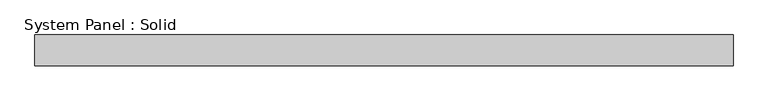
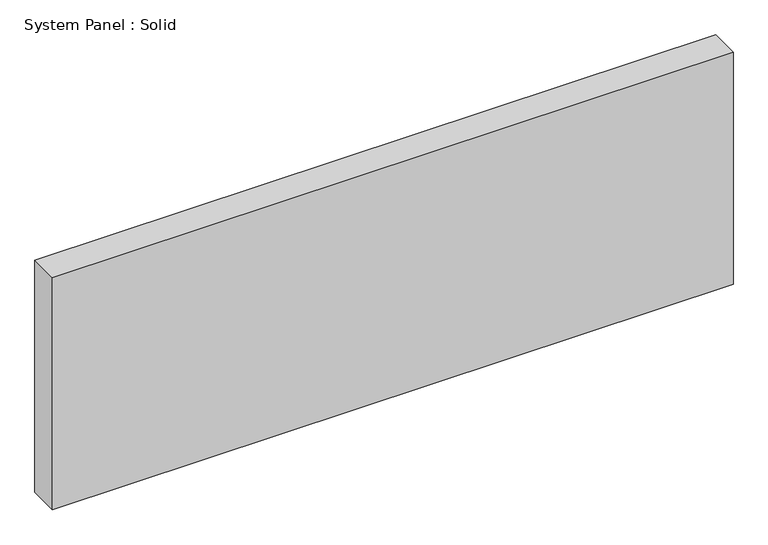
"""IFC4 building model written with IfcOpenShell, lengths in millimetres: plate geometry, System Panel : Solid."""

import ifcopenshell
import ifcopenshell.guid

model = None  # the IFC model being written
_history = None  # IfcOwnerHistory: only IFC2X3 demands one
_inside = {}  # id of a spatial element -> (the spatial element, [elements in it])
_under = {}  # id of a project, library or spatial element -> (it, [spatial elements below it])
_declared = {}  # id of a project -> (the project, [libraries it declares])
_typed = {}  # id of a type object -> (the type object, [elements of that type])
_made_of = {}  # id of a material, layer set ... -> (it, [elements and type objects made of it])


def new_model(schema):
    """Start an empty IFC model of exactly this schema.

    Asked for "IFC4X3", IfcOpenShell would pick the latest addendum, in which some entities
    have other attributes; the version numbers below select the first issue.
    IFC2X3 requires an IfcOwnerHistory on every rooted entity: one is made here for all.
    """
    global model, _history
    if schema == "IFC4X3":
        model = ifcopenshell.file(schema_version=(4, 3, 0, 0))
    else:
        model = ifcopenshell.file(schema=schema)
    _inside.clear()
    _under.clear()
    _declared.clear()
    _typed.clear()
    _made_of.clear()
    _history = None
    if model.schema == "IFC2X3":
        org = make("IfcOrganization", Name="unknown")
        user = make(
            "IfcPersonAndOrganization",
            ThePerson=make("IfcPerson", FamilyName="unknown"),
            TheOrganization=org,
        )
        app = make(
            "IfcApplication",
            ApplicationDeveloper=org,
            Version="unknown",
            ApplicationFullName="unknown",
            ApplicationIdentifier="unknown",
        )
        _history = make(
            "IfcOwnerHistory",
            OwningUser=user,
            OwningApplication=app,
            ChangeAction="ADDED",
            CreationDate=0,
        )
    return model


def make(cls, **values):
    """One entity of the class cls with the attributes given. An attribute that is None is left unset."""
    return model.create_entity(
        cls, **{name: value for name, value in values.items() if value is not None}
    )


def rooted(cls, **values):
    """An entity with a GlobalId (a new one), such as an element, a storey or a relation."""
    return make(cls, GlobalId=ifcopenshell.guid.new(), OwnerHistory=_history, **values)


def si_unit(unit_type, name, prefix=None):
    """IfcSIUnit, for example si_unit("LENGTHUNIT", "METRE", prefix="MILLI")."""
    return make("IfcSIUnit", UnitType=unit_type, Prefix=prefix, Name=name)


def assignment(units):
    """IfcUnitAssignment: the units of a project."""
    return None if units is None else make("IfcUnitAssignment", Units=units)


def point(xyz):
    """IfcCartesianPoint."""
    return None if xyz is None else make("IfcCartesianPoint", Coordinates=xyz)


def direction(xyz):
    """IfcDirection."""
    return None if xyz is None else make("IfcDirection", DirectionRatios=xyz)


def frame(location, z_axis=None, x_axis=None):
    """IfcAxis2Placement3D, a coordinate frame: its origin and axes. An axis left out is left unset."""
    return make(
        "IfcAxis2Placement3D",
        Location=point(location),
        Axis=direction(z_axis),
        RefDirection=direction(x_axis),
    )


def origin():
    """The frame at (0, 0, 0) with its axes left unset."""
    return frame((0.0, 0.0, 0.0))


def origin_with_axes():
    """The frame at (0, 0, 0) with the z axis (0, 0, 1) and the x axis (1, 0, 0) written out."""
    return frame((0.0, 0.0, 0.0), z_axis=(0.0, 0.0, 1.0), x_axis=(1.0, 0.0, 0.0))


def place(relative_to, where):
    """IfcLocalPlacement: puts the frame where relative to a parent placement (None: the world)."""
    return make(
        "IfcLocalPlacement", PlacementRelTo=relative_to, RelativePlacement=where
    )


def context(
    kind, dimensions, precision=None, world=None, true_north=None, identifier=None
):
    """IfcGeometricRepresentationContext, for example the 3D "Model" context."""
    return make(
        "IfcGeometricRepresentationContext",
        ContextIdentifier=identifier,
        ContextType=kind,
        CoordinateSpaceDimension=dimensions,
        Precision=precision,
        WorldCoordinateSystem=world,
        TrueNorth=true_north,
    )


def project(units=None, contexts=None):
    """IfcProject with its units and contexts."""
    return rooted(
        "IfcProject",
        Name="project",
        RepresentationContexts=contexts,
        UnitsInContext=assignment(units),
    )


def spatial(cls, under=None, at=None, **own):
    """A site, building, storey or space (cls), placed at a placement, below another one or the project."""
    s = rooted(cls, ObjectPlacement=at, **own)
    if under is not None:
        _under.setdefault(under.id(), (under, []))[1].append(s)
    return s


def polyline(points):
    """IfcPolyline through the points."""
    return make("IfcPolyline", Points=[point(p) for p in points])


def outline(outer, holes=None, kind="AREA"):
    """IfcArbitraryClosedProfileDef: a profile drawn as a closed curve; with holes, ...WithVoids."""
    if holes is None:
        return make("IfcArbitraryClosedProfileDef", ProfileType=kind, OuterCurve=outer)
    return make(
        "IfcArbitraryProfileDefWithVoids",
        ProfileType=kind,
        OuterCurve=outer,
        InnerCurves=holes,
    )


def extrude(swept, where, along, depth):
    """IfcExtrudedAreaSolid: the profile swept, set in the frame where, extruded along a direction by depth."""
    return make(
        "IfcExtrudedAreaSolid",
        SweptArea=swept,
        Position=where,
        ExtrudedDirection=direction(along),
        Depth=depth,
    )


def shape(context_of_items, identifier, shape_type, items):
    """IfcShapeRepresentation: the items that make up one representation, for example the "Body"."""
    return make(
        "IfcShapeRepresentation",
        ContextOfItems=context_of_items,
        RepresentationIdentifier=identifier,
        RepresentationType=shape_type,
        Items=items,
    )


def source(mapping_origin, context_of_items, identifier, shape_type, items):
    """IfcRepresentationMap: a shape defined once, which mapped items show again and again."""
    return make(
        "IfcRepresentationMap",
        MappingOrigin=mapping_origin,
        MappedRepresentation=shape(context_of_items, identifier, shape_type, items),
    )


def transform(
    local_origin,
    x_axis=None,
    y_axis=None,
    z_axis=None,
    scale=None,
    scale2=None,
    scale3=None,
    uniform=True,
):
    """IfcCartesianTransformationOperator3D, or its non-uniform kind. x_axis, y_axis, z_axis: its Axis1, 2, 3."""
    if uniform:
        return make(
            "IfcCartesianTransformationOperator3D",
            Axis1=direction(x_axis),
            Axis2=direction(y_axis),
            LocalOrigin=point(local_origin),
            Scale=scale,
            Axis3=direction(z_axis),
        )
    return make(
        "IfcCartesianTransformationOperator3DnonUniform",
        Axis1=direction(x_axis),
        Axis2=direction(y_axis),
        LocalOrigin=point(local_origin),
        Scale=scale,
        Axis3=direction(z_axis),
        Scale2=scale2,
        Scale3=scale3,
    )


def mapped(mapping_source, mapping_target):
    """IfcMappedItem: shows the shape of a source again, moved by a transform."""
    return make(
        "IfcMappedItem", MappingSource=mapping_source, MappingTarget=mapping_target
    )


def made_of(thing, what):
    """Note that an element or type object is made of a material, layer set ...; save() writes the relation."""
    if what is not None:
        _made_of.setdefault(what.id(), (what, []))[1].append(thing)
    return thing


def element(
    cls,
    number,
    at=None,
    inside=None,
    cuts=None,
    type_object=None,
    material=None,
    context=None,
    identifier="Body",
    shape_type=None,
    held_by="IfcProductDefinitionShape",
    body=None,
    shapes=None,
    **own,
):
    """One element of the class cls, such as IfcWall. Its Tag is "e" and its number.

    at: its placement. inside: the storey or other place that contains it. cuts: it is an
    opening in that element (IfcRelVoidsElement). A single representation is given by context,
    identifier, shape_type and body (its items); several are given by shapes. held_by: the class
    of the entity that holds the representations. save() writes the other relations.
    """
    e = rooted(cls, Tag="e%d" % number, ObjectPlacement=at, **own)
    if body is not None:
        shapes = [shape(context, identifier, shape_type, body)]
    if shapes is not None:
        e.Representation = make(held_by, Representations=shapes)
    if inside is not None:
        _inside.setdefault(inside.id(), (inside, []))[1].append(e)
    if cuts is not None:
        rooted(
            "IfcRelVoidsElement", RelatingBuildingElement=cuts, RelatedOpeningElement=e
        )
    if type_object is not None:
        _typed.setdefault(type_object.id(), (type_object, []))[1].append(e)
    return made_of(e, material)


def aggregate(whole, parts):
    """IfcRelAggregates: a whole, such as a stair, and the parts it consists of."""
    return rooted("IfcRelAggregates", RelatingObject=whole, RelatedObjects=parts)


def save(model, path):
    """Write the relations noted so far, then the file.

    IfcRelAggregates (storeys below a building ...), IfcRelContainedInSpatialStructure (elements
    in a storey), IfcRelDefinesByType, IfcRelAssociatesMaterial and IfcRelDeclares: one each for
    every whole, place, type object, material and project.
    """
    for whole, parts in _under.values():
        aggregate(whole, parts)
    for where, things in _inside.values():
        rooted(
            "IfcRelContainedInSpatialStructure",
            RelatedElements=things,
            RelatingStructure=where,
        )
    for kind, things in _typed.values():
        rooted("IfcRelDefinesByType", RelatedObjects=things, RelatingType=kind)
    for what, things in _made_of.values():
        rooted("IfcRelAssociatesMaterial", RelatedObjects=things, RelatingMaterial=what)
    for by, libraries in _declared.values():
        rooted("IfcRelDeclares", RelatingContext=by, RelatedDefinitions=libraries)
    model.write(path)


def system_panel_solid_81598777(model_context):
    return source(origin(), model_context, "Body", "SweptSolid", [
        extrude(outline(polyline([(713.3166666, -44.45), (-713.3166666, -44.45), (-713.3166666, 19.05), (713.3166666, 19.05), (713.3166666, -44.45)])), origin_with_axes(), (0.0, 0.0, 1.0), 514.35),
    ])


if __name__ == "__main__":
    model = new_model("IFC4")
    model_context = context("Model", 3, world=origin())
    ifc_project = project(units=[si_unit("LENGTHUNIT", "METRE", prefix="MILLI")], contexts=[model_context])
    site = spatial("IfcSite", under=ifc_project)
    building = spatial("IfcBuilding", under=site)
    placement = place(None, origin())
    system_panel_solid_shape = system_panel_solid_81598777(model_context)
    element("IfcPlate", 1, ObjectType="System Panel : Solid", at=placement, inside=building, context=model_context, shape_type="MappedRepresentation", body=[
        mapped(system_panel_solid_shape, transform((0.0, 0.0, 0.0), x_axis=(1.0, 0.0, 0.0), y_axis=(0.0, 1.0, 0.0), z_axis=(0.0, 0.0, 1.0))),
    ])
    save(model, "model.ifc")

# Revit data of these elements
# Type "System Panel : Solid"
#   Construction Type Id = "MDOOR"
#   Analytic Construction = "Metal"
#   Visual Light Transmittance = 0
#   Solar Heat Gain Coefficient = 0
#   Heat Transfer Coefficient (U) = 0.651978 BTU/(h·ft²·°F)
#   Define Thermal Properties by = 1
# Element 1 (IfcPlate, "System Panel : Solid")
#   Materials on its faces: "Default"
# Materials
#   "Default": class "Miscellaneous", colour RGB 127 127 127, transparency 0, Cost = 0
